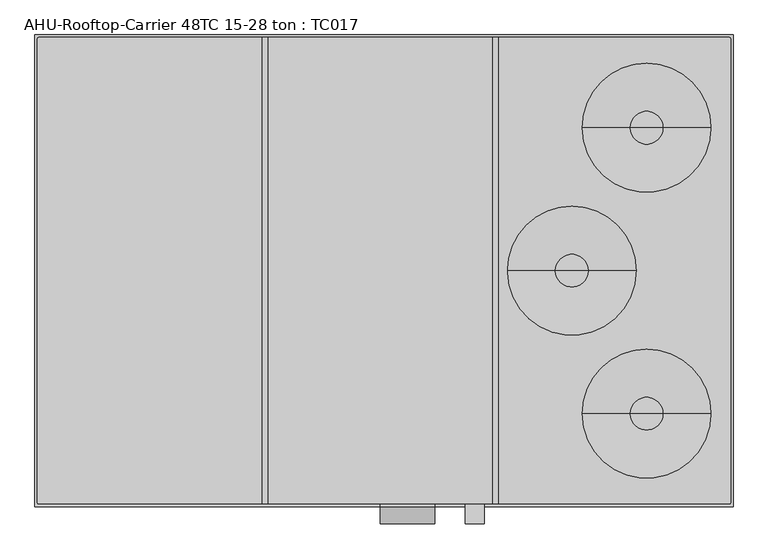
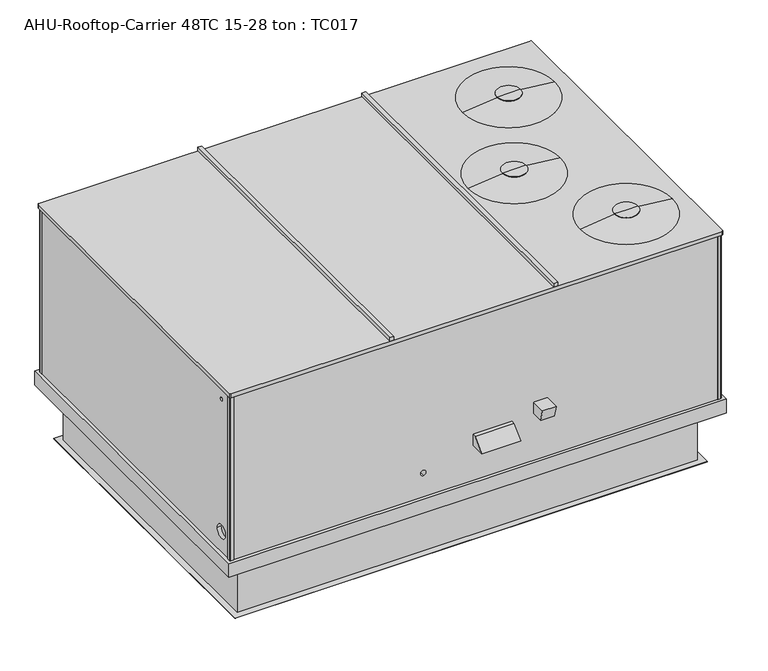
"""IFC4 building model written with IfcOpenShell, lengths in millimetres: proxy geometry, AHU-Rooftop-Carrier 48TC 15-28 ton : TC017."""

from ifc_helpers import new_model, si_unit, point, frame, frame_2d, origin, place, context, project, spatial, polyline, circle_curve, trimmed, segment, composite_curve, outline, extrude, faceted_brep, source, transform, mapped, element, save
from ifc_brep_helpers import plane_surface, cylinder_surface, revolved_surface, advanced_brep


def ahu_rooftop_carrier_48tc_15_28_ton_tc017_cd20dceb(model_context):
    return source(origin(), model_context, "Body", "SolidModel", [
        extrude(outline(composite_curve([segment(trimmed(circle_curve(frame_2d((1605.75625, 1078.70625)), 6.35), [point((1605.75625, 1085.05625))], [point((1612.10625, 1078.70625))], False, "CARTESIAN"), True, "CONTINUOUS"), segment(polyline([(1612.10625, 1078.70625), (1612.10625, -1078.70625)]), True, "CONTINUOUS"), segment(trimmed(circle_curve(frame_2d((1605.75625, -1078.70625)), 6.35), [point((1612.10625, -1078.70625))], [point((1605.75625, -1085.05625))], False, "CARTESIAN"), True, "CONTINUOUS"), segment(polyline([(1605.75625, -1085.05625), (-1605.75625, -1085.05625)]), True, "CONTINUOUS"), segment(trimmed(circle_curve(frame_2d((-1605.75625, -1078.70625)), 6.35), [point((-1605.75625, -1085.05625))], [point((-1612.10625, -1078.70625))], False, "CARTESIAN"), True, "CONTINUOUS"), segment(polyline([(-1612.10625, -1078.70625), (-1612.10625, 1078.70625)]), True, "CONTINUOUS"), segment(trimmed(circle_curve(frame_2d((-1605.75625, 1078.70625)), 6.35), [point((-1612.10625, 1078.70625))], [point((-1605.75625, 1085.05625))], False, "CARTESIAN"), True, "CONTINUOUS"), segment(polyline([(-1605.75625, 1085.05625), (1605.75625, 1085.05625)]), True, "CONTINUOUS")], self_intersect=False)), frame((0.0, 0.0, 1584.325), z_axis=(0.0, 0.0, 1.0), x_axis=(1.0, 0.0, 0.0)), (0.0, 0.0, 1.0), 25.4),
        extrude(outline(polyline([(1624.0125, -1096.9625), (-1624.0125, -1096.9625), (-1624.0125, 1096.9625), (1624.0125, 1096.9625), (1624.0125, -1096.9625)])), frame((0.0, 0.0, 355.6), z_axis=(0.0, 0.0, 1.0), x_axis=(1.0, 0.0, 0.0)), (0.0, 0.0, 1.0), 95.25),
        faceted_brep([(1544.6375, 1023.9375, 355.6), (-1544.6375, 1023.9375, 355.6), (-1544.6375, -1023.9375, 355.6), (1544.6375, -1023.9375, 355.6), (-933.45, 979.4875, 355.6), (-933.45, -787.4, 355.6), (-1498.6, -787.4, 355.6), (-1498.6, 979.4875, 355.6), (388.9375, 976.3125, 355.6), (388.9375, -646.1125, 355.6), (-319.0875, -646.1125, 355.6), (-319.0875, 976.3125, 355.6), (1544.6375, 1023.9375, 0.0), (1544.6375, -1023.9375, 0.0), (-1544.6375, -1023.9375, 0.0), (-1544.6375, 1023.9375, 0.0), (-933.45, 979.4875, 0.0), (-1498.6, 979.4875, 0.0), (-1498.6, -787.4, 0.0), (-933.45, -787.4, 0.0), (388.9375, 976.3125, 0.0), (-319.0875, 976.3125, 0.0), (-319.0875, -646.1125, 0.0), (388.9375, -646.1125, 0.0), (1544.6375, 1023.9375, 330.2), (-1544.6375, 1023.9375, 330.2), (-1544.6375, 1023.9375, 3.175), (1544.6375, 1023.9375, 3.175), (-1544.6375, -1023.9375, 330.2), (-1544.6375, -1023.9375, 3.175), (1544.6375, -1023.9375, 330.2), (1544.6375, -1023.9375, 3.175), (1503.3625, 982.6625, 330.2), (-1503.3625, 982.6625, 330.2), (-1503.3625, -982.6625, 330.2), (1503.3625, -982.6625, 330.2), (1503.3625, 982.6625, 3.175), (1503.3625, -982.6625, 3.175), (-1503.3625, -982.6625, 3.175), (-1503.3625, 982.6625, 3.175)], [[[0, 1, 2, 3], [4, 5, 6, 7], [8, 9, 10, 11]], [[12, 13, 14, 15], [16, 17, 18, 19], [20, 21, 22, 23]], [[1, 0, 24, 25]], [[12, 15, 26, 27]], [[2, 1, 25, 28]], [[15, 14, 29, 26]], [[3, 2, 28, 30]], [[14, 13, 31, 29]], [[0, 3, 30, 24]], [[13, 12, 27, 31]], [[25, 24, 30, 28], [32, 33, 34, 35]], [[27, 26, 29, 31], [36, 37, 38, 39]], [[32, 35, 37, 36]], [[35, 34, 38, 37]], [[34, 33, 39, 38]], [[33, 32, 36, 39]], [[5, 4, 16, 19]], [[6, 5, 19, 18]], [[7, 6, 18, 17]], [[4, 7, 17, 16]], [[9, 8, 20, 23]], [[10, 9, 23, 22]], [[11, 10, 22, 21]], [[8, 11, 21, 20]]]),
        extrude(outline(polyline([(-976.3125, 938.2125), (-976.3125, -792.1625), (-1465.2625, -792.1625), (-1465.2625, 938.2125), (-976.3125, 938.2125)])), frame((0.0, 0.0, 330.2), z_axis=(0.0, 0.0, 1.0), x_axis=(1.0, 0.0, 0.0)), (0.0, 0.0, 1.0), 25.4),
        extrude(outline(polyline([(-258.7625, 938.2125), (388.9375, 938.2125), (388.9375, -627.0625), (-258.7625, -627.0625), (-258.7625, 938.2125)])), frame((0.0, 0.0, 330.2), z_axis=(0.0, 0.0, 1.0), x_axis=(1.0, 0.0, 0.0)), (0.0, 0.0, 1.0), 25.4),
        advanced_brep(
        [(1580.35625, 1075.53125, 1584.325), (-1580.35625, 1075.53125, 1584.325), (-1580.35625, 1053.30625, 1584.325), (-1602.58125, 1053.30625, 1584.325), (-1602.58125, -1053.30625, 1584.325), (-1580.35625, -1053.30625, 1584.325), (-1580.35625, -1075.53125, 1584.325), (1580.35625, -1075.53125, 1584.325), (1580.35625, -1053.30625, 1584.325), (1602.58125, -1053.30625, 1584.325), (1602.58125, 1053.30625, 1584.325), (1580.35625, 1053.30625, 1584.325), (1580.35625, 1075.53125, 450.85), (1580.35625, 1053.30625, 450.85), (1602.58125, 1053.30625, 450.85), (1602.58125, -1053.30625, 450.85), (1580.35625, -1053.30625, 450.85), (1580.35625, -1075.53125, 450.85), (-1580.35625, -1075.53125, 450.85), (-1580.35625, -1053.30625, 450.85), (-1602.58125, -1053.30625, 450.85), (-1602.58125, 1053.30625, 450.85), (-1580.35625, 1053.30625, 450.85), (-1580.35625, 1075.53125, 450.85), (-671.5125, 1075.53125, 511.175), (-671.5125, 1075.53125, 466.725), (-1602.58125, -1022.35, 593.725), (-1602.58125, -930.275, 593.725), (-1602.58125, -987.425, 1508.125), (-1602.58125, -965.2, 1508.125), (-341.3125, -1075.53125, 597.9914062), (-341.3125, -1075.53125, 633.9085937), (-671.5125, 944.5625, 466.725), (-671.5125, 944.5625, 511.175), (-1577.18125, -1022.35, 593.725), (-1577.18125, -930.275, 593.725), (-1577.18125, -987.425, 1508.125), (-1577.18125, -965.2, 1508.125), (-341.3125, -1001.7125, 597.9914062), (-341.3125, -1001.7125, 633.9085937)],
        [
            (0, 1),
            (1, 2),
            (2, 3),
            (3, 4),
            (4, 5),
            (5, 6),
            (6, 7),
            (7, 8),
            (8, 9),
            (9, 10),
            (10, 11),
            (11, 0),
            (12, 13),
            (13, 14),
            (14, 15),
            (15, 16),
            (16, 17),
            (17, 18),
            (18, 19),
            (19, 20),
            (20, 21),
            (21, 22),
            (22, 23),
            (23, 12),
            (0, 12),
            (23, 1),
            (24, 25, circle_curve(frame((-671.5125, 1075.53125, 488.95), z_axis=(0.0, -1.0, 0.0), x_axis=(0.0, 0.0, 1.0)), 22.225)),
            (25, 24, circle_curve(frame((-671.5125, 1075.53125, 488.95), z_axis=(0.0, -1.0, 0.0), x_axis=(0.0, 0.0, 1.0)), 22.225)),
            (22, 2),
            (21, 3),
            (20, 4),
            (26, 27, circle_curve(frame((-1602.58125, -976.3125, 593.725), z_axis=(1.0, 0.0, 0.0), x_axis=(0.0, 1.0, 0.0)), 46.0375)),
            (27, 26, circle_curve(frame((-1602.58125, -976.3125, 593.725), z_axis=(1.0, 0.0, 0.0), x_axis=(0.0, 1.0, 0.0)), 46.0375)),
            (28, 29, circle_curve(frame((-1602.58125, -976.3125, 1508.125), z_axis=(1.0, 0.0, 0.0), x_axis=(0.0, 1.0, 0.0)), 11.1125)),
            (29, 28, circle_curve(frame((-1602.58125, -976.3125, 1508.125), z_axis=(1.0, 0.0, 0.0), x_axis=(0.0, 1.0, 0.0)), 11.1125)),
            (19, 5),
            (18, 6),
            (17, 7),
            (30, 31, circle_curve(frame((-341.3125, -1075.53125, 615.95), z_axis=(0.0, 1.0, 0.0), x_axis=(0.0, 0.0, 1.0)), 17.9585938)),
            (31, 30, circle_curve(frame((-341.3125, -1075.53125, 615.95), z_axis=(0.0, 1.0, 0.0), x_axis=(0.0, 0.0, 1.0)), 17.9585938)),
            (16, 8),
            (15, 9),
            (14, 10),
            (13, 11),
            (32, 33, circle_curve(frame((-671.5125, 944.5625, 488.95), z_axis=(0.0, 1.0, 0.0), x_axis=(0.0, 0.0, 1.0)), 22.225)),
            (33, 32, circle_curve(frame((-671.5125, 944.5625, 488.95), z_axis=(0.0, 1.0, 0.0), x_axis=(0.0, 0.0, 1.0)), 22.225)),
            (32, 25),
            (24, 33),
            (34, 35, circle_curve(frame((-1577.18125, -976.3125, 593.725), z_axis=(-1.0, 0.0, 0.0), x_axis=(0.0, 1.0, 0.0)), 46.0375)),
            (35, 34, circle_curve(frame((-1577.18125, -976.3125, 593.725), z_axis=(-1.0, 0.0, 0.0), x_axis=(0.0, 1.0, 0.0)), 46.0375)),
            (36, 37, circle_curve(frame((-1577.18125, -976.3125, 1508.125), z_axis=(-1.0, 0.0, 0.0), x_axis=(0.0, 1.0, 0.0)), 11.1125)),
            (37, 36, circle_curve(frame((-1577.18125, -976.3125, 1508.125), z_axis=(-1.0, 0.0, 0.0), x_axis=(0.0, 1.0, 0.0)), 11.1125)),
            (35, 27),
            (26, 34),
            (37, 29),
            (28, 36),
            (38, 39, circle_curve(frame((-341.3125, -1001.7125, 615.95), z_axis=(0.0, -1.0, 0.0), x_axis=(0.0, 0.0, 1.0)), 17.9585937)),
            (39, 38, circle_curve(frame((-341.3125, -1001.7125, 615.95), z_axis=(0.0, -1.0, 0.0), x_axis=(0.0, 0.0, 1.0)), 17.9585938)),
            (39, 31),
            (30, 38),
        ],
        [
            plane_surface(frame((-1580.35625, 1075.53125, 1584.325), z_axis=(0.0, 0.0, 1.0), x_axis=(-1.0, 0.0, 0.0))),
            plane_surface(frame((-1580.35625, 1075.53125, 450.85), z_axis=(0.0, 0.0, -1.0), x_axis=(1.0, 0.0, 0.0))),
            plane_surface(frame((1580.35625, 1075.53125, 1584.325), z_axis=(0.0, 1.0, 0.0), x_axis=(0.0, 0.0, -1.0))),
            plane_surface(frame((-1580.35625, 1075.53125, 1584.325), z_axis=(-1.0, 0.0, 0.0), x_axis=(0.0, 0.0, -1.0))),
            plane_surface(frame((-1580.35625, 1053.30625, 1584.325), z_axis=(0.0, 1.0, 0.0), x_axis=(0.0, 0.0, -1.0))),
            plane_surface(frame((-1602.58125, 1053.30625, 1584.325), z_axis=(-1.0, 0.0, 0.0), x_axis=(0.0, 0.0, -1.0))),
            plane_surface(frame((-1602.58125, -1053.30625, 1584.325), z_axis=(0.0, -1.0, 0.0), x_axis=(0.0, 0.0, -1.0))),
            plane_surface(frame((-1580.35625, -1053.30625, 1584.325), z_axis=(-1.0, 0.0, 0.0), x_axis=(0.0, 0.0, -1.0))),
            plane_surface(frame((-1580.35625, -1075.53125, 1584.325), z_axis=(0.0, -1.0, 0.0), x_axis=(0.0, 0.0, -1.0))),
            plane_surface(frame((1580.35625, -1075.53125, 1584.325), z_axis=(1.0, 0.0, 0.0), x_axis=(0.0, 0.0, -1.0))),
            plane_surface(frame((1580.35625, -1053.30625, 1584.325), z_axis=(0.0, -1.0, 0.0), x_axis=(0.0, 0.0, -1.0))),
            plane_surface(frame((1602.58125, -1053.30625, 1584.325), z_axis=(1.0, 0.0, 0.0), x_axis=(0.0, 0.0, -1.0))),
            plane_surface(frame((1602.58125, 1053.30625, 1584.325), z_axis=(0.0, 1.0, 0.0), x_axis=(0.0, 0.0, -1.0))),
            plane_surface(frame((1580.35625, 1053.30625, 1584.325), z_axis=(1.0, 0.0, 0.0), x_axis=(0.0, 0.0, -1.0))),
            plane_surface(frame((-671.5125, 944.5625, 511.175), z_axis=(0.0, 1.0, 0.0), x_axis=(-1.0, 0.0, 0.0))),
            revolved_surface(polyline([(-671.5125, 1075.53125, 511.175), (-671.5125, 944.5625, 511.175)]), (-671.5125, 944.5625, 488.95), (0.0, 1.0, 0.0)),
            plane_surface(frame((-1577.18125, -930.275, 593.725), z_axis=(-1.0, 0.0, 0.0), x_axis=(0.0, 0.0, 1.0))),
            revolved_surface(polyline([(-1577.18125, -930.275, 593.725), (-1602.58125, -930.275, 593.725)]), (-1602.58125, -976.3125, 593.725), (1.0, 0.0, 0.0)),
            revolved_surface(polyline([(-1577.18125, -965.2, 1508.125), (-1602.58125, -965.2, 1508.125)]), (-1602.58125, -976.3125, 1508.125), (1.0, 0.0, 0.0)),
            plane_surface(frame((-341.3125, -1001.7125, 633.9085937), z_axis=(0.0, -1.0, 0.0), x_axis=(1.0, 0.0, 0.0))),
            revolved_surface(polyline([(-341.3125, -1001.7125, 633.9085938000001), (-341.3125, -1075.53125, 633.9085938000001)]), (-341.3125, -1096.9625, 615.95), (0.0, 1.0, 0.0)),
        ],
        [
            (0, [[1, 2, 3, 4, 5, 6, 7, 8, 9, 10, 11, 12]]),
            (1, [[13, 14, 15, 16, 17, 18, 19, 20, 21, 22, 23, 24]]),
            (2, [[-1, 25, -24, 26], [27, 28]]),
            (3, [[-2, -26, -23, 29]]),
            (4, [[-3, -29, -22, 30]]),
            (5, [[-4, -30, -21, 31], [32, 33], [34, 35]]),
            (6, [[-5, -31, -20, 36]]),
            (7, [[-6, -36, -19, 37]]),
            (8, [[-7, -37, -18, 38], [39, 40]]),
            (9, [[-8, -38, -17, 41]]),
            (10, [[-9, -41, -16, 42]]),
            (11, [[-10, -42, -15, 43]]),
            (12, [[-11, -43, -14, 44]]),
            (13, [[-12, -44, -13, -25]]),
            (14, [[45, 46]]),
            (15, [[-45, 47, -27, 48]]),
            (15, [[-46, -48, -28, -47]]),
            (16, [[49, 50]]),
            (16, [[51, 52]]),
            (17, [[-50, 53, -32, 54]]),
            (17, [[-49, -54, -33, -53]]),
            (18, [[-52, 55, -34, 56]]),
            (18, [[-51, -56, -35, -55]]),
            (19, [[57, 58]]),
            (20, [[-58, 59, -39, 60]]),
            (20, [[-57, -60, -40, -59]]),
        ],
    ),
        advanced_brep(
        [(1145.38125, 665.1625, 1635.125), (1297.78125, 665.1625, 1635.125), (1297.78125, 665.1625, 1638.3), (1145.38125, 665.1625, 1638.3), (916.78125, 665.1625, 1609.725), (1526.38125, 665.1625, 1609.725), (1221.58125, 665.1625, 1609.725), (1221.58125, 665.1625, 1638.3)],
        [
            (0, 1, circle_curve(frame((1221.58125, 665.1625, 1635.125), z_axis=(0.0, 0.0, 1.0), x_axis=(1.0, 0.0, 0.0)), 76.2)),
            (1, 2),
            (2, 3, circle_curve(frame((1221.58125, 665.1625, 1638.3), z_axis=(0.0, 0.0, -1.0), x_axis=(1.0, 0.0, 0.0)), 76.2)),
            (3, 0),
            (1, 0, circle_curve(frame((1221.58125, 665.1625, 1635.125), z_axis=(0.0, 0.0, 1.0), x_axis=(1.0, 0.0, 0.0)), 76.2)),
            (3, 2, circle_curve(frame((1221.58125, 665.1625, 1638.3), z_axis=(0.0, 0.0, -1.0), x_axis=(1.0, 0.0, 0.0)), 76.2)),
            (4, 5, circle_curve(frame((1221.58125, 665.1625, 1609.725), z_axis=(0.0, 0.0, 1.0), x_axis=(1.0, 0.0, 0.0)), 304.8)),
            (5, 1),
            (0, 4),
            (5, 4, circle_curve(frame((1221.58125, 665.1625, 1609.725), z_axis=(0.0, 0.0, 1.0), x_axis=(1.0, 0.0, 0.0)), 304.8)),
            (6, 5),
            (4, 6),
            (2, 7),
            (7, 3),
        ],
        [
            cylinder_surface(frame((1221.58125, 665.1625, 1758.8546504), z_axis=(0.0, 0.0, -1.0), x_axis=(1.0, 0.0, 0.0)), 76.2),
            revolved_surface(polyline([(1297.78125, 665.1625, 1635.125), (1526.38125, 665.1625, 1609.725)]), (1221.58125, 665.1625, 1758.8546504), (0.0, 0.0, -1.0)),
            plane_surface(frame((1221.58125, 665.1625, 1609.725), z_axis=(0.0, 0.0, -1.0), x_axis=(1.0, 0.0, 0.0))),
            plane_surface(frame((1221.58125, 665.1625, 1638.3), z_axis=(0.0, 0.0, 1.0), x_axis=(1.0, 0.0, 0.0))),
        ],
        [
            (0, [[1, 2, 3, 4]]),
            (0, [[5, -4, 6, -2]]),
            (1, [[7, 8, -1, 9]]),
            (1, [[10, -9, -5, -8]]),
            (2, [[11, -7, 12]]),
            (2, [[-12, -10, -11]]),
            (3, [[-3, 13, 14]]),
            (3, [[-6, -14, -13]]),
        ],
    ),
        advanced_brep(
        [(797.71875, 0.0, 1635.125), (950.11875, 0.0, 1635.125), (950.11875, 0.0, 1638.3), (797.71875, 0.0, 1638.3), (569.11875, 0.0, 1609.725), (1178.71875, 0.0, 1609.725), (873.91875, 0.0, 1609.725), (873.91875, 0.0, 1638.3)],
        [
            (0, 1, circle_curve(frame((873.91875, 0.0, 1635.125), z_axis=(0.0, 0.0, 1.0), x_axis=(1.0, 0.0, 0.0)), 76.2)),
            (1, 2),
            (2, 3, circle_curve(frame((873.91875, 0.0, 1638.3), z_axis=(0.0, 0.0, -1.0), x_axis=(1.0, 0.0, 0.0)), 76.2)),
            (3, 0),
            (1, 0, circle_curve(frame((873.91875, 0.0, 1635.125), z_axis=(0.0, 0.0, 1.0), x_axis=(1.0, 0.0, 0.0)), 76.2)),
            (3, 2, circle_curve(frame((873.91875, 0.0, 1638.3), z_axis=(0.0, 0.0, -1.0), x_axis=(1.0, 0.0, 0.0)), 76.2)),
            (4, 5, circle_curve(frame((873.91875, 0.0, 1609.725), z_axis=(0.0, 0.0, 1.0), x_axis=(1.0, 0.0, 0.0)), 304.8)),
            (5, 1),
            (0, 4),
            (5, 4, circle_curve(frame((873.91875, 0.0, 1609.725), z_axis=(0.0, 0.0, 1.0), x_axis=(1.0, 0.0, 0.0)), 304.8)),
            (6, 5),
            (4, 6),
            (2, 7),
            (7, 3),
        ],
        [
            cylinder_surface(frame((873.91875, 0.0, 1758.8546504), z_axis=(0.0, 0.0, -1.0), x_axis=(1.0, 0.0, 0.0)), 76.2),
            revolved_surface(polyline([(950.11875, 0.0, 1635.125), (1178.71875, 0.0, 1609.725)]), (873.91875, 0.0, 1758.8546504), (0.0, 0.0, -1.0)),
            plane_surface(frame((873.91875, 0.0, 1609.725), z_axis=(0.0, 0.0, -1.0), x_axis=(1.0, 0.0, 0.0))),
            plane_surface(frame((873.91875, 0.0, 1638.3), z_axis=(0.0, 0.0, 1.0), x_axis=(1.0, 0.0, 0.0))),
        ],
        [
            (0, [[1, 2, 3, 4]]),
            (0, [[5, -4, 6, -2]]),
            (1, [[7, 8, -1, 9]]),
            (1, [[10, -9, -5, -8]]),
            (2, [[11, -7, 12]]),
            (2, [[-12, -10, -11]]),
            (3, [[-3, 13, 14]]),
            (3, [[-6, -14, -13]]),
        ],
    ),
        advanced_brep(
        [(1145.38125, -665.1625, 1635.125), (1297.78125, -665.1625, 1635.125), (1297.78125, -665.1625, 1638.3), (1145.38125, -665.1625, 1638.3), (916.78125, -665.1625, 1609.725), (1526.38125, -665.1625, 1609.725), (1221.58125, -665.1625, 1609.725), (1221.58125, -665.1625, 1638.3)],
        [
            (0, 1, circle_curve(frame((1221.58125, -665.1625, 1635.125), z_axis=(0.0, 0.0, 1.0), x_axis=(1.0, 0.0, 0.0)), 76.2)),
            (1, 2),
            (2, 3, circle_curve(frame((1221.58125, -665.1625, 1638.3), z_axis=(0.0, 0.0, -1.0), x_axis=(1.0, 0.0, 0.0)), 76.2)),
            (3, 0),
            (1, 0, circle_curve(frame((1221.58125, -665.1625, 1635.125), z_axis=(0.0, 0.0, 1.0), x_axis=(1.0, 0.0, 0.0)), 76.2)),
            (3, 2, circle_curve(frame((1221.58125, -665.1625, 1638.3), z_axis=(0.0, 0.0, -1.0), x_axis=(1.0, 0.0, 0.0)), 76.2)),
            (4, 5, circle_curve(frame((1221.58125, -665.1625, 1609.725), z_axis=(0.0, 0.0, 1.0), x_axis=(1.0, 0.0, 0.0)), 304.8)),
            (5, 1),
            (0, 4),
            (5, 4, circle_curve(frame((1221.58125, -665.1625, 1609.725), z_axis=(0.0, 0.0, 1.0), x_axis=(1.0, 0.0, 0.0)), 304.8)),
            (6, 5),
            (4, 6),
            (2, 7),
            (7, 3),
        ],
        [
            cylinder_surface(frame((1221.58125, -665.1625, 1758.8546504), z_axis=(0.0, 0.0, -1.0), x_axis=(1.0, 0.0, 0.0)), 76.2),
            revolved_surface(polyline([(1297.78125, -665.1625, 1635.125), (1526.38125, -665.1625, 1609.725)]), (1221.58125, -665.1625, 1758.8546504), (0.0, 0.0, -1.0)),
            plane_surface(frame((1221.58125, -665.1625, 1609.725), z_axis=(0.0, 0.0, -1.0), x_axis=(1.0, 0.0, 0.0))),
            plane_surface(frame((1221.58125, -665.1625, 1638.3), z_axis=(0.0, 0.0, 1.0), x_axis=(1.0, 0.0, 0.0))),
        ],
        [
            (0, [[1, 2, 3, 4]]),
            (0, [[5, -4, 6, -2]]),
            (1, [[7, 8, -1, 9]]),
            (1, [[10, -9, -5, -8]]),
            (2, [[11, -7, 12]]),
            (2, [[-12, -10, -11]]),
            (3, [[-3, 13, 14]]),
            (3, [[-6, -14, -13]]),
        ],
    ),
        extrude(outline(composite_curve([segment(polyline([(-1580.35625, 1078.70625), (-1580.35625, 1053.30625), (-1605.75625, 1053.30625), (-1605.75625, 1072.35625)]), True, "CONTINUOUS"), segment(trimmed(circle_curve(frame_2d((-1599.40625, 1072.35625)), 6.35), [point((-1605.75625, 1072.35625))], [point((-1599.40625, 1078.70625))], False, "CARTESIAN"), True, "CONTINUOUS"), segment(polyline([(-1599.40625, 1078.70625), (-1580.35625, 1078.70625)]), True, "CONTINUOUS")], self_intersect=False)), frame((0.0, 0.0, 450.85), z_axis=(0.0, 0.0, 1.0), x_axis=(1.0, 0.0, 0.0)), (0.0, 0.0, 1.0), 1133.475),
        extrude(outline(composite_curve([segment(trimmed(circle_curve(frame_2d((1599.40625, 1072.35625)), 6.35), [point((1599.40625, 1078.70625))], [point((1605.75625, 1072.35625))], False, "CARTESIAN"), True, "CONTINUOUS"), segment(polyline([(1605.75625, 1072.35625), (1605.75625, 1053.30625), (1580.35625, 1053.30625), (1580.35625, 1078.70625), (1599.40625, 1078.70625)]), True, "CONTINUOUS")], self_intersect=False)), frame((0.0, 0.0, 450.85), z_axis=(0.0, 0.0, 1.0), x_axis=(1.0, 0.0, 0.0)), (0.0, 0.0, 1.0), 1133.475),
        extrude(outline(composite_curve([segment(polyline([(1605.75625, -1053.30625), (1605.75625, -1072.35625)]), True, "CONTINUOUS"), segment(trimmed(circle_curve(frame_2d((1599.40625, -1072.35625)), 6.35), [point((1605.75625, -1072.35625))], [point((1599.40625, -1078.70625))], False, "CARTESIAN"), True, "CONTINUOUS"), segment(polyline([(1599.40625, -1078.70625), (1580.35625, -1078.70625), (1580.35625, -1053.30625), (1605.75625, -1053.30625)]), True, "CONTINUOUS")], self_intersect=False)), frame((0.0, 0.0, 450.85), z_axis=(0.0, 0.0, 1.0), x_axis=(1.0, 0.0, 0.0)), (0.0, 0.0, 1.0), 1133.475),
        extrude(outline(composite_curve([segment(polyline([(-1580.35625, -1053.30625), (-1580.35625, -1078.70625), (-1599.40625, -1078.70625)]), True, "CONTINUOUS"), segment(trimmed(circle_curve(frame_2d((-1599.40625, -1072.35625)), 6.35), [point((-1599.40625, -1078.70625))], [point((-1605.75625, -1072.35625))], False, "CARTESIAN"), True, "CONTINUOUS"), segment(polyline([(-1605.75625, -1072.35625), (-1605.75625, -1053.30625), (-1580.35625, -1053.30625)]), True, "CONTINUOUS")], self_intersect=False)), frame((0.0, 0.0, 450.85), z_axis=(0.0, 0.0, 1.0), x_axis=(1.0, 0.0, 0.0)), (0.0, 0.0, 1.0), 1133.475),
        extrude(outline(polyline([(-1075.53125, 695.325), (-1177.13125, 695.325), (-1100.93125, 771.525), (-1075.53125, 771.525), (-1075.53125, 695.325)])), frame((-17.2640625, 0.0, 0.0), z_axis=(1.0, 0.0, 0.0), x_axis=(0.0, 1.0, 0.0)), (0.0, 0.0, 1.0), 254.0),
        extrude(outline(polyline([(-1075.53125, 777.875), (-1158.08125, 777.875), (-1177.13125, 854.075), (-1075.53125, 854.075), (-1075.53125, 777.875)])), frame((378.61875, 0.0, 0.0), z_axis=(1.0, 0.0, 0.0), x_axis=(0.0, 1.0, 0.0)), (0.0, 0.0, 1.0), 88.9),
        extrude(outline(polyline([(-540.146875, 1085.05625), (-540.146875, -1085.05625), (-565.546875, -1085.05625), (-565.546875, 1085.05625), (-540.146875, 1085.05625)])), frame((0.0, 0.0, 1609.725), z_axis=(0.0, 0.0, 1.0), x_axis=(1.0, 0.0, 0.0)), (0.0, 0.0, 1.0), 25.4),
        extrude(outline(polyline([(531.01875, 1085.05625), (531.01875, -1085.05625), (505.61875, -1085.05625), (505.61875, 1085.05625), (531.01875, 1085.05625)])), frame((0.0, 0.0, 1609.725), z_axis=(0.0, 0.0, 1.0), x_axis=(1.0, 0.0, 0.0)), (0.0, 0.0, 1.0), 25.4),
    ])


if __name__ == "__main__":
    model = new_model("IFC4")
    model_context = context("Model", 3, world=origin())
    ifc_project = project(units=[si_unit("LENGTHUNIT", "METRE", prefix="MILLI")], contexts=[model_context])
    site = spatial("IfcSite", under=ifc_project)
    building = spatial("IfcBuilding", under=site)
    placement = place(None, origin())
    ahu_rooftop_carrier_48tc_15_28_ton_tc017_shape = ahu_rooftop_carrier_48tc_15_28_ton_tc017_cd20dceb(model_context)
    element("IfcBuildingElementProxy", 1, Name="AHU-Rooftop-Carrier 48TC 15-28 ton : TC017", ObjectType="AHU-Rooftop-Carrier 48TC 15-28 ton : TC017", at=placement, inside=building, context=model_context, shape_type="MappedRepresentation", body=[
        mapped(ahu_rooftop_carrier_48tc_15_28_ton_tc017_shape, transform((0.0, 0.0, 0.0), x_axis=(1.0, 0.0, 0.0), y_axis=(0.0, 1.0, 0.0), z_axis=(0.0, 0.0, 1.0))),
    ])
    save(model, "model.ifc")

# Revit data of these elements
# Type "AHU-Rooftop-Carrier 48TC 15-28 ton : TC017"
#   URL = "www.carrier.com"
#   Manufacturer = "Carrier"
#   Description = "48TC WeatherExpert Series Ultra High Efficient Single Package Rooftop and Single Zone VAV Cooling Only with Optional Electric Heat with Puron (R-410A) Refrigerant \r\nUltra High Efficient\r\nSingle Package Rooftop and Single Zone VAV Cooling Only with Optional Electric Heat with Puron (R-410A) Refrigerant"
#   Assembly Code = "D3050200"
#   Voltage [instance default] = 240 V
#   Unit Width = 7' - 0 15/16"
#   Unit Size = 17
#   Unit Length = 10' - 6 7/16"
#   Unit Height = 4' - 1 3/8"
#   Supply Air Width V = 61 5/8"
#   Supply Air Width Label 2 [instance default] = 61 5/8"
#   Supply Air Width Label [instance default] = -61 5/8"
#   Supply Air Width H = 29 3/4"
#   Supply Air Height V = 25 1/2"
#   Supply Air Height Label [instance default] = 25 1/2"
#   Supply Air Height H = 15 7/8"
#   SA Z Offset = 0' - 5 5/8"
#   SA Y Offset Label [instance default] = 6' - 8 1/8"
#   SA Y Offset V = 0' - 6 1/4"
#   SA Y Offset H = 0' - 0 23/32"
#   SA X Offset Label [instance default] = 4' - 0 5/8"
#   SA X Offset V = 4' - 5 3/4"
#   SA X Offset H = 4' - 2 3/4"
#   Return Air Width V = 19 1/4"
#   Return Air Width Label 3 [instance default] = -1' - 7 1/4"
#   Return Air Width Label 2 [instance default] = 19 1/4"
#   Return Air Width Label [instance default] = 19 1/4"
#   Return Air Width H = 23 3/8"
#   Return Air Height V = 68 1/8"
#   Return Air Height Label [instance default] = 68 1/8"
#   Return Air Height H = 41 3/8"
#   Return Air Flow [instance default] = 0 CFM
#   RA Z Offset = 0' - 5 5/8"
#   RA Y Offset V = 0' - 6 1/4"
#   RA Y Offset Label [instance default] = 1' - 0"
#   RA Y Offset H = 0' - 0 23/32"
#   RA X Offset V = 0' - 6 1/4"
#   RA X Offset Label [instance default] = 8' - 6 3/8"
#   RA X Offset H = 0' - 3 1/4"
#   Power Z Offset = 0' - 9 3/8"
#   Power Y Offset = 0' - 4 3/4"
#   Power Knockout Radius = 0' - 1 13/16"
#   Power Factor [instance default] = 0.8
#   Power Exhaust Width = 1' - 5"
#   Power Exhaust Offset = 1' - 5"
#   Power Exhaust Length = 3' - 7"
#   Power Exhaust Height = 1' - 11"
#   Pivot Y = 6' - 0"
#   Pivot X = 12' - 0"
#   Supply Air Nominal Capacity [instance default] = 0 CFM
#   Length 9 = 0' - 11 7/8"
#   Length 8 [instance default] = 0' - 0"
#   Length 7 [instance default] = 0' - 0"
#   Length 6 [instance default] = 0' - 1"
#   Length 5 = 4' - 2"
#   Length 4 = 3' - 6 11/64"
#   Length 3 = 7' - 0 11/32"
#   Length 2 = 0' - 0 1/4"
#   Length 15 = 1' - 4 11/128"
#   Length 14 = 0' - 2"
#   Length 13 [instance default] = -5' - 1 5/8"
#   Length 12 = 3' - 6 11/64"
#   Length 11 = 2' - 4.11458"
#   Length 10 = 7' - 0 11/32"
#   Length 1 [instance default] = 1' - 2"
#   Grille Radius = 1' - 0"
#   Grille Cover Radius = 0' - 3"
#   Grille 6 Y Offset = 0' - 0"
#   Grille 6 X Offset = 0' - 0"
#   Grille 5 Y Offset = 0' - 0"
#   Grille 5 X Offset = 0' - 0"
#   Grille 4 Y Offset = 5' - 9 3/8"
#   Grille 4 X Offset = 9' - 4 1/32"
#   Grille 3 Y Offset = 3' - 7 3/16"
#   Grille 3 X Offset = 8' - 2 11/32"
#   Grille 2 Y Offset = 3' - 7 3/16"
#   Grille 2 X Offset = 10' - 5 23/32"
#   Grille 1 X Offset = 9' - 4 1/32"
#   Grille 1 Y Offset = 1' - 5"
#   Gas Z Offset Label [instance default] = 0' - 10 1/4"
#   Gas Z Offset = 0' - 10 1/4"
#   Gas Y Offset Label [instance default] = 0' - 0"
#   Gas Y Offset = 0' - 6 1/2"
#   Gas X Offset = 4' - 2 1/2"
#   Gas Radius [instance default] = 3/8"
#   Gas Pressure Drop [instance default] = 0.00 psi
#   Gas Knockout Radius [instance default] = 0' - 0 181/256"
#   Gas Flow [instance default] = 0 GPM
#   Frame Width = 0' - 1"
#   Fan Height = 0' - 1 1/8"
#   Economizer Z Offset V = 4' - 0 1/4"
#   Economizer Z Offset Label [instance default] = 4' - 0 1/4"
#   Economizer Z Offset H = 3' - 7 1/4"
#   Economizer Y Offset = 1' - 2 1/8"
#   Economizer X Offset = 0' - 3"
#   Economizer Width V = 2' - 0 7/8"
#   Economizer Width Label [instance default] = 2' - 0 7/8"
#   Economizer Width H = 2' - 0 7/8"
#   Economizer Length V = 5' - 8"
#   Economizer Length Label [instance default] = 5' - 8"
#   Economizer Length H = 5' - 8"
#   Economizer Height V = 2' - 5 1/4"
#   Economizer Height Label [instance default] = 2' - 5 1/4"
#   Economizer Height H = 2' - 0 1/4"
#   Drain Z Offset Label [instance default] = 0' - 5 1/4"
#   Drain Z Offset = 0' - 5 1/4"
#   Drain Y Offset V = 0' - 0"
#   Drain Y Offset Label [instance default] = 7' - 2 3/8"
#   Drain Y Offset H = 0' - 0"
#   Drain X Offset Label [instance default] = 7' - 6 3/8"
#   Drain X Offset = 3' - 1 1/2"
#   Drain Radius [instance default] = 3/8"
#   Drain Knockout Radius [instance default] = 0' - 0 7/8"
#   Curb Width = 6' - 8 5/8"
#   Curb SA Y Offset = 1' - 1 1/8"
#   Curb SA X Offset = 3' - 7 3/4"
#   Curb SA Width = 2' - 3 7/8"
#   Curb SA Height = 5' - 3 7/8"
#   Curb RA Y Offset = 0' - 0"
#   Curb RA X Offset = 7' - 11 13/16"
#   Curb RA Width = 1' - 10 1/4"
#   Curb RA Height = 5' - 9 9/16"
#   Curb Offset Y Label = 6' - 0"
#   Curb Offset Y = 0' - 0"
#   Curb Offset X Label = 12' - 0"
#   Curb Offset X = 0' - 0"
#   Curb Length = 10' - 1 5/8"
#   Curb Height Label [instance default] = 1' - 2"
#   Curb Height 2 = 2' - 0"
#   Curb Height 1 = 1' - 2"
#   Nominal Capacity = 180000.0 Btu/h
#   Control Z Offset = 3' - 9 3/8"
#   Control Y Offset = 0' - 4 3/4"
#   Control Knockout Radius = 0' - 0 7/16"
#   Clearance Right [instance default] = 1' - 6"
#   Clearance Left [instance default] = 1' - 0"
#   Clearance Front [instance default] = 3' - 0"
#   Clearance Back [instance default] = 3' - 0"
#   Base Width = 7' - 2 3/8"
#   Base Length = 10' - 7 7/8"
#   Base Height = 0' - 3 3/4"
#   Apparent Load [instance default] = 0 VA
#   Angle 9 [instance default] = 90.00°
#   Angle 8 [instance default] = 90.00°
#   Angle 7 = 180.00°
#   Angle 6 [instance default] = 0.00°
#   Angle 5 [instance default] = 180.00°
#   Angle 4 [instance default] = 0.00°
#   Angle 3 [instance default] = 270.00°
#   Angle 2 [instance default] = 50.00°
#   Angle 1 [instance default] = 0.00°
#   Air Pressure Drop [instance default] = 0.00 in-wg
#   Visibility Power Exhaust [instance default] = no
#   Visibility Horizontal Air [instance default] = no
#   Visibility Horizontal Air End Unit [instance default] = no
#   Visibility Gas Alternate [instance default] = no
#   Visibility Economizer [instance default] = no
#   Visibility Drain Alternate [instance default] = no
#   Visibility 9 [instance default] = no
#   Visibility 8 [instance default] = no
#   Visibility 7 [instance default] = no
#   Visibility 6 [instance default] = no
#   Visibility 5 = yes
#   Visibility 4 = no
#   Visibility 3 = yes
#   Visibility 2 [instance default] = yes
#   Visibility 12 = no
#   Visibility 11 [instance default] = yes
#   Visibility 10 [instance default] = no
#   Visibility 1 = yes
#   Vertical Air [instance default] = yes
#   Roof Curb 24" [instance default] = no
#   Roof Curb 14" [instance default] = yes
#   Power Exhaust [instance default] = no
#   Number of Poles [instance default] = 1
#   Horizontal Air End Unit [instance default] = no
#   Horizontal Air = no
#   Gas Alternate [instance default] = no
#   Economizer or 2 Position Damper [instance default] = no
#   Economizer Vertical [instance default] = no
#   Economizer Horizontal [instance default] = no
#   Drain Alternate = no
#   Clearance Zones [instance default] = no
#   Load Classification [instance default] = HVAC
#   Grille Material = Metal - Carrier - Grille
#   Curb Material = Metal - Carrier - Steel
#   Clearance Material = Clearance Zones - Carrier
#   Body Material = RTU
#   Base Material = Metal - Carrier - Stainless Steel
# Element 1 (IfcBuildingElementProxy, "AHU-Rooftop-Carrier 48TC 15-28 ton : TC017")
#   Clearance Right = 3' - 0"
#   Clearance Left = 3' - 6"
#   Clearance Front = 3' - 6"
#   Clearance Back = 3' - 6"
#   Materials on its faces: "RTU", "Metal - Carrier - Steel", "Metal - Carrier - Grille", "Metal - Carrier - Stainless Steel"
# Materials
#   "Metal - Carrier - Grille": class "Miscellaneous", colour RGB 93 90 88, transparency 0
#   "Metal - Carrier - Steel": class "Miscellaneous", colour RGB 192 192 192, transparency 0
#   "Clearance Zones - Carrier": class "Unassigned", colour RGB 255 0 0, transparency 0.85
#   "RTU": class "Miscellaneous", colour RGB 104 104 104, transparency 0, Cost = 0
#   "Metal - Carrier - Stainless Steel": class "Miscellaneous", colour RGB 189 187 185, transparency 0
